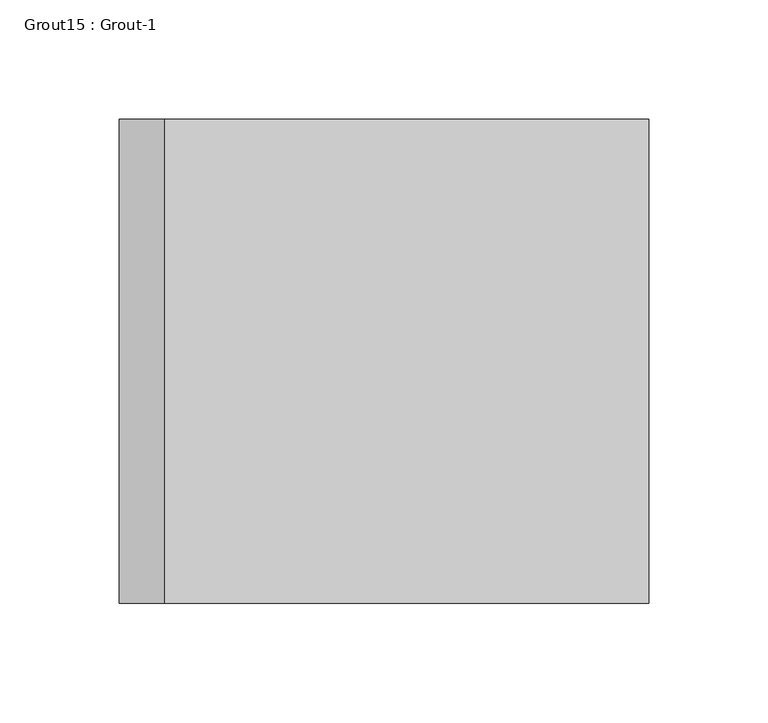
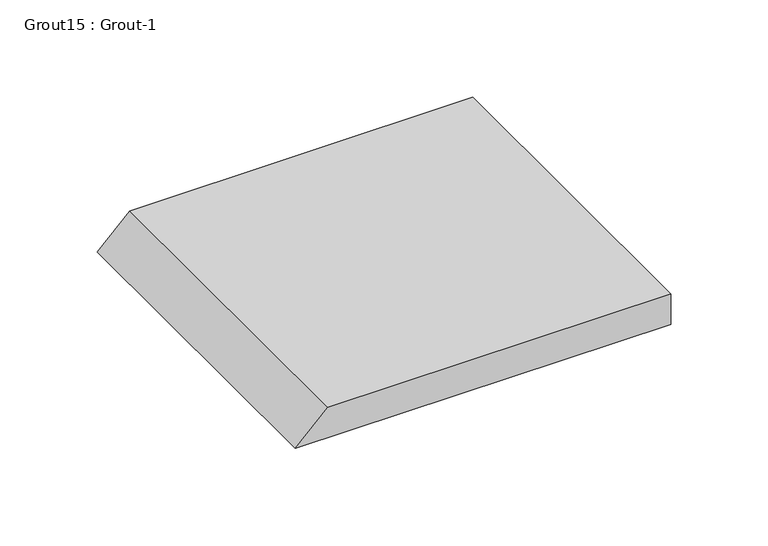
"""IFC4 building model written with IfcOpenShell, lengths in millimetres: proxy geometry, Grout15 : Grout-1."""

from ifc_helpers import new_model, si_unit, frame, origin, place, context, project, spatial, polyline, outline, extrude, source, transform, mapped, element, save


def grout15_grout_1_4b3d9b04(model_context):
    return source(origin(), model_context, "Body", "SweptSolid", [
        extrude(outline(polyline([(19.05, 590115.4434739), (0.0, 590096.3934739), (0.0, 590318.6434739), (19.05, 590318.6434739), (19.05, 590115.4434739)])), frame((0.0, -532982.2413841, 0.0), z_axis=(0.0, 1.0, 0.0), x_axis=(0.0, 0.0, 1.0)), (0.0, 0.0, 1.0), 203.2),
    ])


if __name__ == "__main__":
    model = new_model("IFC4")
    model_context = context("Model", 3, world=origin())
    ifc_project = project(units=[si_unit("LENGTHUNIT", "METRE", prefix="MILLI")], contexts=[model_context])
    site = spatial("IfcSite", under=ifc_project)
    building = spatial("IfcBuilding", under=site)
    placement = place(None, origin())
    grout15_grout_1_shape = grout15_grout_1_4b3d9b04(model_context)
    element("IfcBuildingElementProxy", 1, Name="Grout15 : Grout-1", ObjectType="Grout15 : Grout-1", at=placement, inside=building, context=model_context, shape_type="MappedRepresentation", body=[
        mapped(grout15_grout_1_shape, transform((0.0, 0.0, 0.0), x_axis=(1.0, 0.0, 0.0), y_axis=(0.0, 1.0, 0.0), z_axis=(0.0, 0.0, 1.0))),
    ])
    save(model, "model.ifc")

# Revit data of these elements
# Element 1 (IfcBuildingElementProxy, "Grout15 : Grout-1")
#   Materials on its faces: "3/4\" NON SHRINK GROUT"
# Materials
#   "3/4\" NON SHRINK GROUT": class "Generic", colour RGB 145 145 143, transparency 0, Cost = 0
